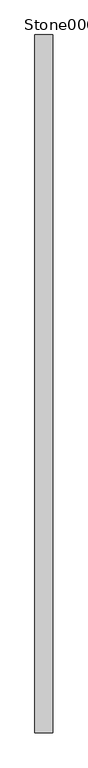
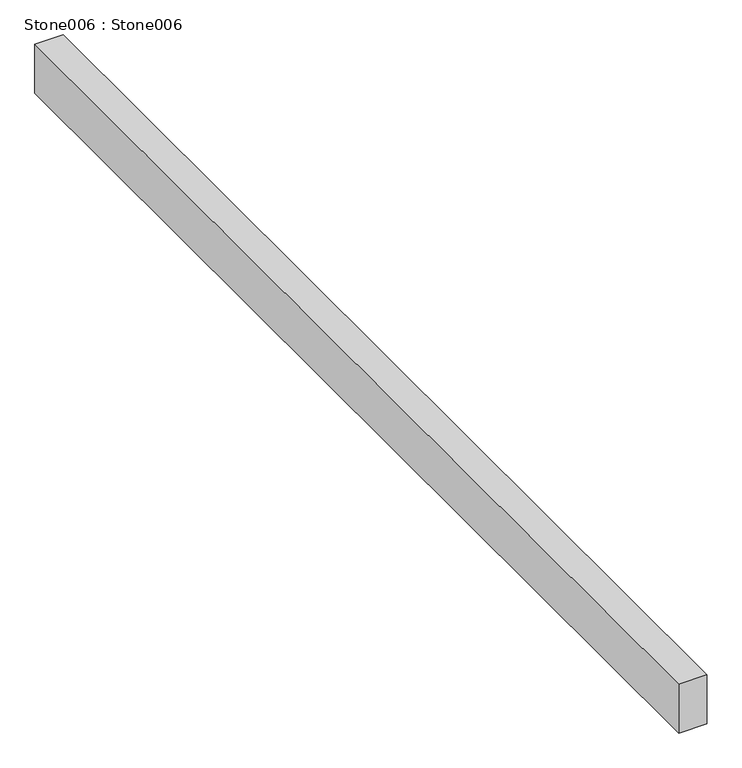
"""IFC4 building model written with IfcOpenShell, lengths in millimetres: proxy geometry, Stone006 : Stone006."""

from ifc_helpers import new_model, si_unit, frame, origin, place, context, project, spatial, polyline, outline, extrude, source, transform, mapped, element, save


def stone006_stone006_c00c7167(model_context):
    return source(origin(), model_context, "Body", "SweptSolid", [
        extrude(outline(polyline([(-6063.6492306, -1052.8906574), (-6114.4492306, -1052.8906574), (-6114.4492306, 947.1093426), (-6063.6492306, 947.1093426), (-6063.6492306, -1052.8906574)])), frame((0.0, 0.0, 36406.6444375), z_axis=(0.0, 0.0, 1.0), x_axis=(1.0, 0.0, 0.0)), (0.0, 0.0, 1.0), 92.6719688),
    ])


if __name__ == "__main__":
    model = new_model("IFC4")
    model_context = context("Model", 3, world=origin())
    ifc_project = project(units=[si_unit("LENGTHUNIT", "METRE", prefix="MILLI")], contexts=[model_context])
    site = spatial("IfcSite", under=ifc_project)
    building = spatial("IfcBuilding", under=site)
    placement = place(None, origin())
    stone006_stone006_shape = stone006_stone006_c00c7167(model_context)
    element("IfcBuildingElementProxy", 1, Name="Stone006 : Stone006", ObjectType="Stone006 : Stone006", at=placement, inside=building, context=model_context, shape_type="MappedRepresentation", body=[
        mapped(stone006_stone006_shape, transform((0.0, 0.0, 0.0), x_axis=(1.0, 0.0, 0.0), y_axis=(0.0, 1.0, 0.0), z_axis=(0.0, 0.0, 1.0))),
    ])
    save(model, "model.ifc")

# Revit data of these elements
# Type "Stone006 : Stone006"
#   NameOverride = "Stone006"
# Element 1 (IfcBuildingElementProxy, "Stone006 : Stone006")
#   Materials on its faces: "2\" STONE DECK TBD"
# Materials
#   "2\" STONE DECK TBD": class "Unassigned", colour RGB 199 185 173, transparency 0
